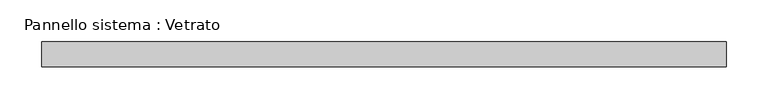
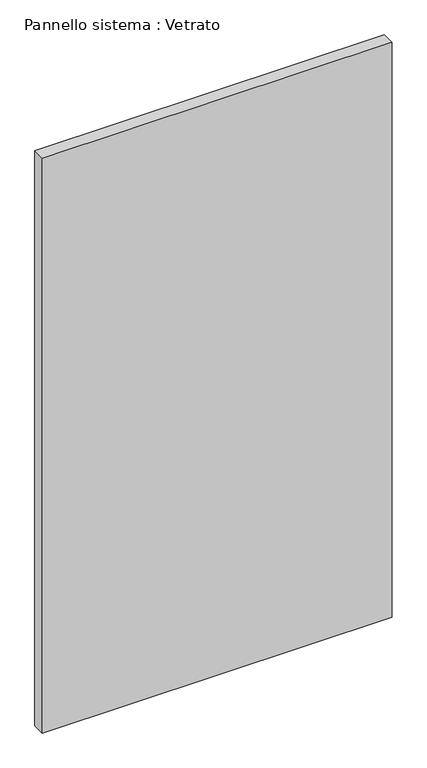
"""IFC4 building model written with IfcOpenShell, lengths in millimetres: plate geometry, Pannello sistema : Vetrato."""

from ifc_helpers import new_model, si_unit, origin, origin_with_axes, place, context, project, spatial, polyline, outline, extrude, source, transform, mapped, element, save


def pannello_sistema_vetrato_501d2436(model_context):
    return source(origin(), model_context, "Body", "SweptSolid", [
        extrude(outline(polyline([(410.0, -15.0), (-410.0, -15.0), (-410.0, 15.0), (410.0, 15.0), (410.0, -15.0)])), origin_with_axes(), (0.0, 0.0, 1.0), 1425.0),
    ])


if __name__ == "__main__":
    model = new_model("IFC4")
    model_context = context("Model", 3, world=origin())
    ifc_project = project(units=[si_unit("LENGTHUNIT", "METRE", prefix="MILLI")], contexts=[model_context])
    site = spatial("IfcSite", under=ifc_project)
    building = spatial("IfcBuilding", under=site)
    placement = place(None, origin())
    pannello_sistema_vetrato_shape = pannello_sistema_vetrato_501d2436(model_context)
    element("IfcPlate", 1, ObjectType="Pannello sistema : Vetrato", at=placement, inside=building, context=model_context, shape_type="MappedRepresentation", body=[
        mapped(pannello_sistema_vetrato_shape, transform((0.0, 0.0, 0.0), x_axis=(1.0, 0.0, 0.0), y_axis=(0.0, 1.0, 0.0), z_axis=(0.0, 0.0, 1.0))),
    ])
    save(model, "model.ifc")

# Revit data of these elements
# Type "Pannello sistema : Vetrato"
#   Construction Type Id = "GSP4R"
#   Analytic Construction = "Vetrata singola Pilkington 1/8 in"
#   Visual Light Transmittance = 0.9
#   Solar Heat Gain Coefficient = 0.86
#   Heat Transfer Coefficient (U) = 6.7069 W/(m²·K)
# Element 1 (IfcPlate, "Pannello sistema : Vetrato")
#   Materials on its faces: "Default - Vetro"
# Materials
#   "Default - Vetro": class "Vetro", colour RGB 208 208 208, transparency 0.7, Cost = 0
